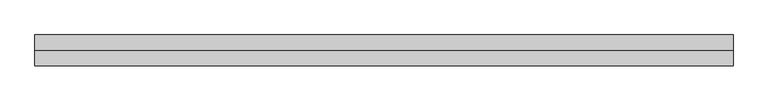
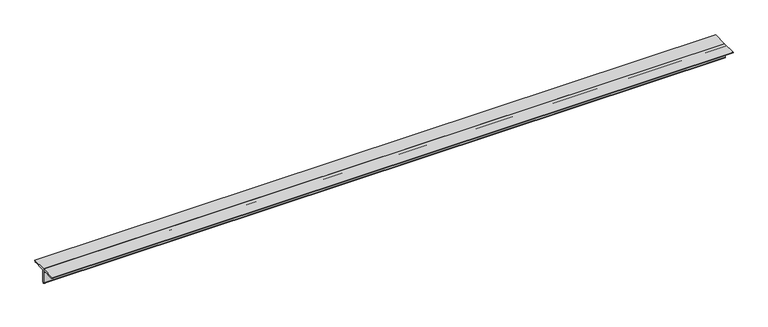
"""IFC4 building model written with IfcOpenShell, lengths in millimetres: member geometry, 0123_Steel Framing_2Ls-KSD3502 : H_SB_AR_S03_2Ls-130x130x12_HBR1."""

from ifc_helpers import new_model, si_unit, point, frame, frame_2d, origin, place, context, project, spatial, polyline, circle_curve, trimmed, segment, composite_curve, outline, extrude, source, transform, mapped, element, save


def member_82c07ad7(model_context):
    return source(origin(), model_context, "Body", "SweptSolid", [
        extrude(outline(composite_curve([segment(polyline([(0.0, 36.4), (130.0, 36.4)]), True, "CONTINUOUS"), segment(trimmed(circle_curve(frame_2d((118.0, 36.4)), 12.0), [point((130.0, 36.4))], [point((118.0, 24.4))], False, "CARTESIAN"), True, "CONTINUOUS"), segment(polyline([(118.0, 24.4), (24.0, 24.4)]), True, "CONTINUOUS"), segment(trimmed(circle_curve(frame_2d((24.0, 12.4)), 12.0), [point((24.0, 24.4))], [point((12.0, 12.4))], True, "CARTESIAN"), True, "CONTINUOUS"), segment(polyline([(12.0, 12.4), (12.0, -81.6)]), True, "CONTINUOUS"), segment(trimmed(circle_curve(frame_2d((0.0, -81.6)), 12.0), [point((12.0, -81.6))], [point((0.0, -93.6))], False, "CARTESIAN"), True, "CONTINUOUS"), segment(polyline([(0.0, -93.6), (0.0, 36.4)]), True, "CONTINUOUS")], self_intersect=False)), frame((-2923.0178496, 0.0, 0.0), z_axis=(1.0, 0.0, 0.0), x_axis=(0.0, 1.0, 0.0)), (0.0, 0.0, 1.0), 5889.8945249),
        extrude(outline(composite_curve([segment(polyline([(0.0, 36.4), (0.0, -93.6)]), True, "CONTINUOUS"), segment(trimmed(circle_curve(frame_2d((0.0, -81.6)), 12.0), [point((0.0, -93.6))], [point((-12.0, -81.6))], False, "CARTESIAN"), True, "CONTINUOUS"), segment(polyline([(-12.0, -81.6), (-12.0, 12.4)]), True, "CONTINUOUS"), segment(trimmed(circle_curve(frame_2d((-24.0, 12.4)), 12.0), [point((-12.0, 12.4))], [point((-24.0, 24.4))], True, "CARTESIAN"), True, "CONTINUOUS"), segment(polyline([(-24.0, 24.4), (-118.0, 24.4)]), True, "CONTINUOUS"), segment(trimmed(circle_curve(frame_2d((-118.0, 36.4)), 12.0), [point((-118.0, 24.4))], [point((-130.0, 36.4))], False, "CARTESIAN"), True, "CONTINUOUS"), segment(polyline([(-130.0, 36.4), (0.0, 36.4)]), True, "CONTINUOUS")], self_intersect=False)), frame((-2923.0178496, 0.0, 0.0), z_axis=(1.0, 0.0, 0.0), x_axis=(0.0, 1.0, 0.0)), (0.0, 0.0, 1.0), 5889.8945249),
    ])


if __name__ == "__main__":
    model = new_model("IFC4")
    model_context = context("Model", 3, world=origin())
    ifc_project = project(units=[si_unit("LENGTHUNIT", "METRE", prefix="MILLI")], contexts=[model_context])
    site = spatial("IfcSite", under=ifc_project)
    building = spatial("IfcBuilding", under=site)
    placement = place(None, origin())
    member_shape = member_82c07ad7(model_context)
    element("IfcMember", 1, ObjectType="0123_Steel Framing_2Ls-KSD3502 : H_SB_AR_S03_2Ls-130x130x12_HBR1", at=placement, inside=building, context=model_context, shape_type="MappedRepresentation", body=[
        mapped(member_shape, transform((0.0, 0.0, 0.0), x_axis=(1.0, 0.0, 0.0), y_axis=(0.0, 1.0, 0.0), z_axis=(0.0, 0.0, 1.0))),
    ])
    save(model, "model.ifc")

# Revit data of these elements
# Type "0123_Steel Framing_2Ls-KSD3502 : H_SB_AR_S03_2Ls-130x130x12_HBR1"
#   Type Mark = "HBR1"
#   Assembly Code = "B10"
#   Legs = "SLBB"
#   W = 8.97
#   Perimeter = 1.04 m²/m
#   Nominal Weight = 46.80 kgf/m
#   Length [instance default] = 1000 mm
#   Space = 0 mm
#   b = 130 mm
#   d = 130 mm
#   t = 12 mm
#   y = 36.4 mm
#   A = 0.005952 m²
#   Structural Material [instance default] = Steel ASTM A36
# Element 1 (IfcMember, "0123_Steel Framing_2Ls-KSD3502 : H_SB_AR_S03_2Ls-130x130x12_HBR1")
#   Materials on its faces: "Steel ASTM A36"
# Materials
#   "Steel ASTM A36": class "Metal", colour RGB 199 199 199, transparency 0, Description = "Structural steel, ASTM A36 Grade B, mill finish", Cost = 0
